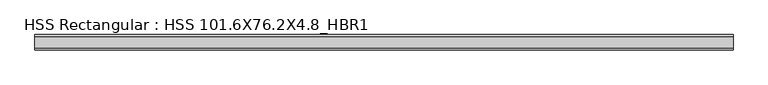
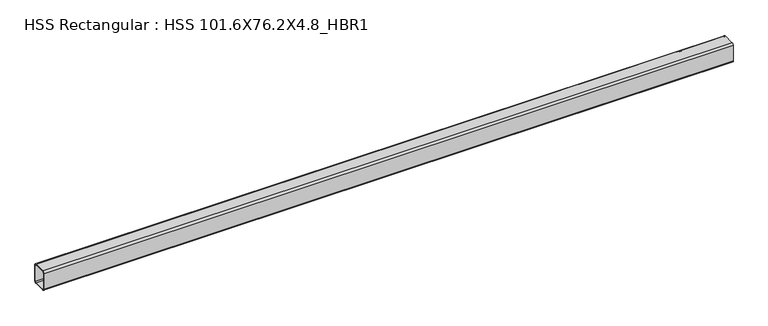
"""IFC4 building model written with IfcOpenShell, lengths in millimetres: beam geometry, HSS Rectangular : HSS 101.6X76.2X4.8_HBR1."""

import ifcopenshell
import ifcopenshell.guid

model = None  # the IFC model being written
_history = None  # IfcOwnerHistory: only IFC2X3 demands one
_inside = {}  # id of a spatial element -> (the spatial element, [elements in it])
_under = {}  # id of a project, library or spatial element -> (it, [spatial elements below it])
_declared = {}  # id of a project -> (the project, [libraries it declares])
_typed = {}  # id of a type object -> (the type object, [elements of that type])
_made_of = {}  # id of a material, layer set ... -> (it, [elements and type objects made of it])


def new_model(schema):
    """Start an empty IFC model of exactly this schema.

    Asked for "IFC4X3", IfcOpenShell would pick the latest addendum, in which some entities
    have other attributes; the version numbers below select the first issue.
    IFC2X3 requires an IfcOwnerHistory on every rooted entity: one is made here for all.
    """
    global model, _history
    if schema == "IFC4X3":
        model = ifcopenshell.file(schema_version=(4, 3, 0, 0))
    else:
        model = ifcopenshell.file(schema=schema)
    _inside.clear()
    _under.clear()
    _declared.clear()
    _typed.clear()
    _made_of.clear()
    _history = None
    if model.schema == "IFC2X3":
        org = make("IfcOrganization", Name="unknown")
        user = make(
            "IfcPersonAndOrganization",
            ThePerson=make("IfcPerson", FamilyName="unknown"),
            TheOrganization=org,
        )
        app = make(
            "IfcApplication",
            ApplicationDeveloper=org,
            Version="unknown",
            ApplicationFullName="unknown",
            ApplicationIdentifier="unknown",
        )
        _history = make(
            "IfcOwnerHistory",
            OwningUser=user,
            OwningApplication=app,
            ChangeAction="ADDED",
            CreationDate=0,
        )
    return model


def make(cls, **values):
    """One entity of the class cls with the attributes given. An attribute that is None is left unset."""
    return model.create_entity(
        cls, **{name: value for name, value in values.items() if value is not None}
    )


def rooted(cls, **values):
    """An entity with a GlobalId (a new one), such as an element, a storey or a relation."""
    return make(cls, GlobalId=ifcopenshell.guid.new(), OwnerHistory=_history, **values)


def si_unit(unit_type, name, prefix=None):
    """IfcSIUnit, for example si_unit("LENGTHUNIT", "METRE", prefix="MILLI")."""
    return make("IfcSIUnit", UnitType=unit_type, Prefix=prefix, Name=name)


def assignment(units):
    """IfcUnitAssignment: the units of a project."""
    return None if units is None else make("IfcUnitAssignment", Units=units)


def point(xyz):
    """IfcCartesianPoint."""
    return None if xyz is None else make("IfcCartesianPoint", Coordinates=xyz)


def direction(xyz):
    """IfcDirection."""
    return None if xyz is None else make("IfcDirection", DirectionRatios=xyz)


def frame(location, z_axis=None, x_axis=None):
    """IfcAxis2Placement3D, a coordinate frame: its origin and axes. An axis left out is left unset."""
    return make(
        "IfcAxis2Placement3D",
        Location=point(location),
        Axis=direction(z_axis),
        RefDirection=direction(x_axis),
    )


def frame_2d(location, x_axis=None):
    """IfcAxis2Placement2D, a coordinate frame in the plane: its origin and x axis."""
    return make(
        "IfcAxis2Placement2D", Location=point(location), RefDirection=direction(x_axis)
    )


def origin():
    """The frame at (0, 0, 0) with its axes left unset."""
    return frame((0.0, 0.0, 0.0))


def place(relative_to, where):
    """IfcLocalPlacement: puts the frame where relative to a parent placement (None: the world)."""
    return make(
        "IfcLocalPlacement", PlacementRelTo=relative_to, RelativePlacement=where
    )


def context(
    kind, dimensions, precision=None, world=None, true_north=None, identifier=None
):
    """IfcGeometricRepresentationContext, for example the 3D "Model" context."""
    return make(
        "IfcGeometricRepresentationContext",
        ContextIdentifier=identifier,
        ContextType=kind,
        CoordinateSpaceDimension=dimensions,
        Precision=precision,
        WorldCoordinateSystem=world,
        TrueNorth=true_north,
    )


def project(units=None, contexts=None):
    """IfcProject with its units and contexts."""
    return rooted(
        "IfcProject",
        Name="project",
        RepresentationContexts=contexts,
        UnitsInContext=assignment(units),
    )


def spatial(cls, under=None, at=None, **own):
    """A site, building, storey or space (cls), placed at a placement, below another one or the project."""
    s = rooted(cls, ObjectPlacement=at, **own)
    if under is not None:
        _under.setdefault(under.id(), (under, []))[1].append(s)
    return s


def polyline(points):
    """IfcPolyline through the points."""
    return make("IfcPolyline", Points=[point(p) for p in points])


def circle_curve(where, radius):
    """IfcCircle in the frame where."""
    return make("IfcCircle", Position=where, Radius=radius)


def trimmed(basis, trim1, trim2, sense, master):
    """IfcTrimmedCurve: the piece of a basis curve between two trims."""
    return make(
        "IfcTrimmedCurve",
        BasisCurve=basis,
        Trim1=trim1,
        Trim2=trim2,
        SenseAgreement=sense,
        MasterRepresentation=master,
    )


def segment(curve, same_sense, transition):
    """IfcCompositeCurveSegment."""
    return make(
        "IfcCompositeCurveSegment",
        Transition=transition,
        SameSense=same_sense,
        ParentCurve=curve,
    )


def composite_curve(segments, self_intersect=None):
    """IfcCompositeCurve: segments joined end to end."""
    return make("IfcCompositeCurve", Segments=segments, SelfIntersect=self_intersect)


def outline(outer, holes=None, kind="AREA"):
    """IfcArbitraryClosedProfileDef: a profile drawn as a closed curve; with holes, ...WithVoids."""
    if holes is None:
        return make("IfcArbitraryClosedProfileDef", ProfileType=kind, OuterCurve=outer)
    return make(
        "IfcArbitraryProfileDefWithVoids",
        ProfileType=kind,
        OuterCurve=outer,
        InnerCurves=holes,
    )


def extrude(swept, where, along, depth):
    """IfcExtrudedAreaSolid: the profile swept, set in the frame where, extruded along a direction by depth."""
    return make(
        "IfcExtrudedAreaSolid",
        SweptArea=swept,
        Position=where,
        ExtrudedDirection=direction(along),
        Depth=depth,
    )


def shape(context_of_items, identifier, shape_type, items):
    """IfcShapeRepresentation: the items that make up one representation, for example the "Body"."""
    return make(
        "IfcShapeRepresentation",
        ContextOfItems=context_of_items,
        RepresentationIdentifier=identifier,
        RepresentationType=shape_type,
        Items=items,
    )


def source(mapping_origin, context_of_items, identifier, shape_type, items):
    """IfcRepresentationMap: a shape defined once, which mapped items show again and again."""
    return make(
        "IfcRepresentationMap",
        MappingOrigin=mapping_origin,
        MappedRepresentation=shape(context_of_items, identifier, shape_type, items),
    )


def transform(
    local_origin,
    x_axis=None,
    y_axis=None,
    z_axis=None,
    scale=None,
    scale2=None,
    scale3=None,
    uniform=True,
):
    """IfcCartesianTransformationOperator3D, or its non-uniform kind. x_axis, y_axis, z_axis: its Axis1, 2, 3."""
    if uniform:
        return make(
            "IfcCartesianTransformationOperator3D",
            Axis1=direction(x_axis),
            Axis2=direction(y_axis),
            LocalOrigin=point(local_origin),
            Scale=scale,
            Axis3=direction(z_axis),
        )
    return make(
        "IfcCartesianTransformationOperator3DnonUniform",
        Axis1=direction(x_axis),
        Axis2=direction(y_axis),
        LocalOrigin=point(local_origin),
        Scale=scale,
        Axis3=direction(z_axis),
        Scale2=scale2,
        Scale3=scale3,
    )


def mapped(mapping_source, mapping_target):
    """IfcMappedItem: shows the shape of a source again, moved by a transform."""
    return make(
        "IfcMappedItem", MappingSource=mapping_source, MappingTarget=mapping_target
    )


def made_of(thing, what):
    """Note that an element or type object is made of a material, layer set ...; save() writes the relation."""
    if what is not None:
        _made_of.setdefault(what.id(), (what, []))[1].append(thing)
    return thing


def element(
    cls,
    number,
    at=None,
    inside=None,
    cuts=None,
    type_object=None,
    material=None,
    context=None,
    identifier="Body",
    shape_type=None,
    held_by="IfcProductDefinitionShape",
    body=None,
    shapes=None,
    **own,
):
    """One element of the class cls, such as IfcWall. Its Tag is "e" and its number.

    at: its placement. inside: the storey or other place that contains it. cuts: it is an
    opening in that element (IfcRelVoidsElement). A single representation is given by context,
    identifier, shape_type and body (its items); several are given by shapes. held_by: the class
    of the entity that holds the representations. save() writes the other relations.
    """
    e = rooted(cls, Tag="e%d" % number, ObjectPlacement=at, **own)
    if body is not None:
        shapes = [shape(context, identifier, shape_type, body)]
    if shapes is not None:
        e.Representation = make(held_by, Representations=shapes)
    if inside is not None:
        _inside.setdefault(inside.id(), (inside, []))[1].append(e)
    if cuts is not None:
        rooted(
            "IfcRelVoidsElement", RelatingBuildingElement=cuts, RelatedOpeningElement=e
        )
    if type_object is not None:
        _typed.setdefault(type_object.id(), (type_object, []))[1].append(e)
    return made_of(e, material)


def aggregate(whole, parts):
    """IfcRelAggregates: a whole, such as a stair, and the parts it consists of."""
    return rooted("IfcRelAggregates", RelatingObject=whole, RelatedObjects=parts)


def save(model, path):
    """Write the relations noted so far, then the file.

    IfcRelAggregates (storeys below a building ...), IfcRelContainedInSpatialStructure (elements
    in a storey), IfcRelDefinesByType, IfcRelAssociatesMaterial and IfcRelDeclares: one each for
    every whole, place, type object, material and project.
    """
    for whole, parts in _under.values():
        aggregate(whole, parts)
    for where, things in _inside.values():
        rooted(
            "IfcRelContainedInSpatialStructure",
            RelatedElements=things,
            RelatingStructure=where,
        )
    for kind, things in _typed.values():
        rooted("IfcRelDefinesByType", RelatedObjects=things, RelatingType=kind)
    for what, things in _made_of.values():
        rooted("IfcRelAssociatesMaterial", RelatedObjects=things, RelatingMaterial=what)
    for by, libraries in _declared.values():
        rooted("IfcRelDeclares", RelatingContext=by, RelatedDefinitions=libraries)
    model.write(path)


def hss_rectangular_hss_101_6x76_2x4_8_hbr1_7f5480d4(model_context):
    return source(origin(), model_context, "Body", "SweptSolid", [
        extrude(outline(composite_curve([segment(polyline([(38.1, 41.275), (38.1, -41.275)]), True, "CONTINUOUS"), segment(trimmed(circle_curve(frame_2d((28.575, -41.275)), 9.525), [point((38.1, -41.275))], [point((28.575, -50.8))], False, "CARTESIAN"), True, "CONTINUOUS"), segment(polyline([(28.575, -50.8), (-28.575, -50.8)]), True, "CONTINUOUS"), segment(trimmed(circle_curve(frame_2d((-28.575, -41.275)), 9.525), [point((-28.575, -50.8))], [point((-38.1, -41.275))], False, "CARTESIAN"), True, "CONTINUOUS"), segment(polyline([(-38.1, -41.275), (-38.1, 41.275)]), True, "CONTINUOUS"), segment(trimmed(circle_curve(frame_2d((-28.575, 41.275)), 9.525), [point((-38.1, 41.275))], [point((-28.575, 50.8))], False, "CARTESIAN"), True, "CONTINUOUS"), segment(polyline([(-28.575, 50.8), (28.575, 50.8)]), True, "CONTINUOUS"), segment(trimmed(circle_curve(frame_2d((28.575, 41.275)), 9.525), [point((28.575, 50.8))], [point((38.1, 41.275))], False, "CARTESIAN"), True, "CONTINUOUS")], self_intersect=False), holes=[composite_curve([segment(trimmed(circle_curve(frame_2d((-28.575, 41.275)), 4.7625), [point((-28.575, 46.0375))], [point((-33.3375, 41.275))], True, "CARTESIAN"), True, "CONTINUOUS"), segment(polyline([(-33.3375, 41.275), (-33.3375, -41.275)]), True, "CONTINUOUS"), segment(trimmed(circle_curve(frame_2d((-28.575, -41.275)), 4.7625), [point((-33.3375, -41.275))], [point((-28.575, -46.0375))], True, "CARTESIAN"), True, "CONTINUOUS"), segment(polyline([(-28.575, -46.0375), (28.575, -46.0375)]), True, "CONTINUOUS"), segment(trimmed(circle_curve(frame_2d((28.575, -41.275)), 4.7625), [point((28.575, -46.0375))], [point((33.3375, -41.275))], True, "CARTESIAN"), True, "CONTINUOUS"), segment(polyline([(33.3375, -41.275), (33.3375, 41.275)]), True, "CONTINUOUS"), segment(trimmed(circle_curve(frame_2d((28.575, 41.275)), 4.7625), [point((33.3375, 41.275))], [point((28.575, 46.0375))], True, "CARTESIAN"), True, "CONTINUOUS"), segment(polyline([(28.575, 46.0375), (-28.575, 46.0375)]), True, "CONTINUOUS")], self_intersect=False)]), frame((-1636.9299526, 0.0, 0.0), z_axis=(1.0, 0.0, 0.0), x_axis=(0.0, 1.0, 0.0)), (0.0, 0.0, 1.0), 3459.2437364),
    ])


if __name__ == "__main__":
    model = new_model("IFC4")
    model_context = context("Model", 3, world=origin())
    ifc_project = project(units=[si_unit("LENGTHUNIT", "METRE", prefix="MILLI")], contexts=[model_context])
    site = spatial("IfcSite", under=ifc_project)
    building = spatial("IfcBuilding", under=site)
    placement = place(None, origin())
    hss_rectangular_hss_101_6x76_2x4_8_hbr1_shape = hss_rectangular_hss_101_6x76_2x4_8_hbr1_7f5480d4(model_context)
    element("IfcBeam", 1, ObjectType="HSS Rectangular : HSS 101.6X76.2X4.8_HBR1", at=placement, inside=building, context=model_context, shape_type="MappedRepresentation", body=[
        mapped(hss_rectangular_hss_101_6x76_2x4_8_hbr1_shape, transform((0.0, 0.0, 0.0), x_axis=(1.0, 0.0, 0.0), y_axis=(0.0, 1.0, 0.0), z_axis=(0.0, 0.0, 1.0))),
    ])
    save(model, "model.ifc")

# Revit data of these elements
# Type "HSS Rectangular : HSS 101.6X76.2X4.8_HBR1"
#   Section Name Key = "HSS 4X3X3/16"
#   Assembly Code = "B10"
#   Width = 7.62 cm
#   Wall Nominal Thickness = 0.4763 cm
#   Wall Design Thickness = 0.442 cm
#   Torsional Moment of Inertia = 260.561 cm⁴
#   Torsional Modulus = 61.2876 cm³
#   Section Area = 14.4516 cm²
#   Plastic Modulus weak axis = 40.3122 cm³
#   Plastic Modulus strong axis = 49.1612 cm³
#   Perimeter = 0.881482 m²/m
#   Outer Fillet = 0.9525 cm
#   Nominal Weight = 12.1285 kgf/m
#   Moment of Inertia weak axis = 131.529 cm⁴
#   Moment of Inertia strong axis = 205.202 cm⁴
#   Inner Fillet = 0.4763 cm
#   Height = 10.16 cm
#   Elastic Modulus weak axis = 34.4128 cm³
#   Elastic Modulus strong axis = 40.476 cm³
#   Centroid Vertical = 5.08 cm
#   Centroid Horizontal = 3.81 cm
#   Length [instance default] = 1524 mm
#   Structural Material [instance default] = Steel ASTM A500, Grade B, Rectangular and Square
#   Principal Axes Angle = 0
# Element 1 (IfcBeam, "HSS Rectangular : HSS 101.6X76.2X4.8_HBR1")
#   Structural Material = Steel ASTM A992
#   Materials on its faces: "Steel ASTM A992"
# Materials
#   "Steel ASTM A500, Grade B, Rectangular and Square": class "Metal", colour RGB 199 199 199, transparency 0, Description = "Carbon steel", Cost = 0
#   "Steel ASTM A992": class "Metal", colour RGB 199 199 199, transparency 0, Description = "Structural steel 50ksi", Cost = 0
